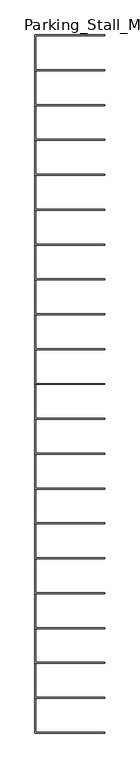
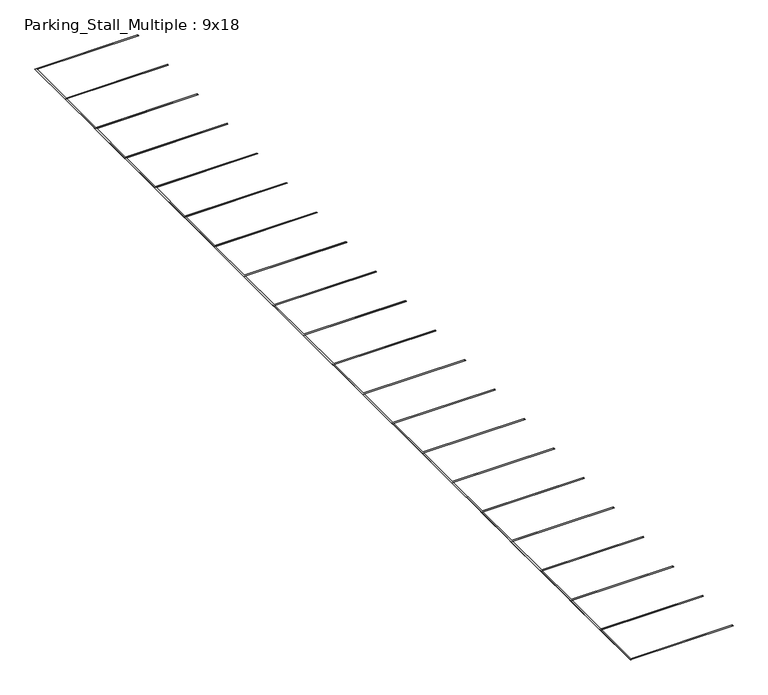
"""IFC4 building model written with IfcOpenShell, lengths in millimetres: proxy geometry, Parking_Stall_Multiple : 9x18."""

import ifcopenshell
import ifcopenshell.guid

model = None  # the IFC model being written
_history = None  # IfcOwnerHistory: only IFC2X3 demands one
_inside = {}  # id of a spatial element -> (the spatial element, [elements in it])
_under = {}  # id of a project, library or spatial element -> (it, [spatial elements below it])
_declared = {}  # id of a project -> (the project, [libraries it declares])
_typed = {}  # id of a type object -> (the type object, [elements of that type])
_made_of = {}  # id of a material, layer set ... -> (it, [elements and type objects made of it])


def new_model(schema):
    """Start an empty IFC model of exactly this schema.

    Asked for "IFC4X3", IfcOpenShell would pick the latest addendum, in which some entities
    have other attributes; the version numbers below select the first issue.
    IFC2X3 requires an IfcOwnerHistory on every rooted entity: one is made here for all.
    """
    global model, _history
    if schema == "IFC4X3":
        model = ifcopenshell.file(schema_version=(4, 3, 0, 0))
    else:
        model = ifcopenshell.file(schema=schema)
    _inside.clear()
    _under.clear()
    _declared.clear()
    _typed.clear()
    _made_of.clear()
    _history = None
    if model.schema == "IFC2X3":
        org = make("IfcOrganization", Name="unknown")
        user = make(
            "IfcPersonAndOrganization",
            ThePerson=make("IfcPerson", FamilyName="unknown"),
            TheOrganization=org,
        )
        app = make(
            "IfcApplication",
            ApplicationDeveloper=org,
            Version="unknown",
            ApplicationFullName="unknown",
            ApplicationIdentifier="unknown",
        )
        _history = make(
            "IfcOwnerHistory",
            OwningUser=user,
            OwningApplication=app,
            ChangeAction="ADDED",
            CreationDate=0,
        )
    return model


def make(cls, **values):
    """One entity of the class cls with the attributes given. An attribute that is None is left unset."""
    return model.create_entity(
        cls, **{name: value for name, value in values.items() if value is not None}
    )


def rooted(cls, **values):
    """An entity with a GlobalId (a new one), such as an element, a storey or a relation."""
    return make(cls, GlobalId=ifcopenshell.guid.new(), OwnerHistory=_history, **values)


def si_unit(unit_type, name, prefix=None):
    """IfcSIUnit, for example si_unit("LENGTHUNIT", "METRE", prefix="MILLI")."""
    return make("IfcSIUnit", UnitType=unit_type, Prefix=prefix, Name=name)


def assignment(units):
    """IfcUnitAssignment: the units of a project."""
    return None if units is None else make("IfcUnitAssignment", Units=units)


def point(xyz):
    """IfcCartesianPoint."""
    return None if xyz is None else make("IfcCartesianPoint", Coordinates=xyz)


def direction(xyz):
    """IfcDirection."""
    return None if xyz is None else make("IfcDirection", DirectionRatios=xyz)


def frame(location, z_axis=None, x_axis=None):
    """IfcAxis2Placement3D, a coordinate frame: its origin and axes. An axis left out is left unset."""
    return make(
        "IfcAxis2Placement3D",
        Location=point(location),
        Axis=direction(z_axis),
        RefDirection=direction(x_axis),
    )


def origin():
    """The frame at (0, 0, 0) with its axes left unset."""
    return frame((0.0, 0.0, 0.0))


def origin_with_axes():
    """The frame at (0, 0, 0) with the z axis (0, 0, 1) and the x axis (1, 0, 0) written out."""
    return frame((0.0, 0.0, 0.0), z_axis=(0.0, 0.0, 1.0), x_axis=(1.0, 0.0, 0.0))


def place(relative_to, where):
    """IfcLocalPlacement: puts the frame where relative to a parent placement (None: the world)."""
    return make(
        "IfcLocalPlacement", PlacementRelTo=relative_to, RelativePlacement=where
    )


def context(
    kind, dimensions, precision=None, world=None, true_north=None, identifier=None
):
    """IfcGeometricRepresentationContext, for example the 3D "Model" context."""
    return make(
        "IfcGeometricRepresentationContext",
        ContextIdentifier=identifier,
        ContextType=kind,
        CoordinateSpaceDimension=dimensions,
        Precision=precision,
        WorldCoordinateSystem=world,
        TrueNorth=true_north,
    )


def project(units=None, contexts=None):
    """IfcProject with its units and contexts."""
    return rooted(
        "IfcProject",
        Name="project",
        RepresentationContexts=contexts,
        UnitsInContext=assignment(units),
    )


def spatial(cls, under=None, at=None, **own):
    """A site, building, storey or space (cls), placed at a placement, below another one or the project."""
    s = rooted(cls, ObjectPlacement=at, **own)
    if under is not None:
        _under.setdefault(under.id(), (under, []))[1].append(s)
    return s


def polyline(points):
    """IfcPolyline through the points."""
    return make("IfcPolyline", Points=[point(p) for p in points])


def outline(outer, holes=None, kind="AREA"):
    """IfcArbitraryClosedProfileDef: a profile drawn as a closed curve; with holes, ...WithVoids."""
    if holes is None:
        return make("IfcArbitraryClosedProfileDef", ProfileType=kind, OuterCurve=outer)
    return make(
        "IfcArbitraryProfileDefWithVoids",
        ProfileType=kind,
        OuterCurve=outer,
        InnerCurves=holes,
    )


def extrude(swept, where, along, depth):
    """IfcExtrudedAreaSolid: the profile swept, set in the frame where, extruded along a direction by depth."""
    return make(
        "IfcExtrudedAreaSolid",
        SweptArea=swept,
        Position=where,
        ExtrudedDirection=direction(along),
        Depth=depth,
    )


def shape(context_of_items, identifier, shape_type, items):
    """IfcShapeRepresentation: the items that make up one representation, for example the "Body"."""
    return make(
        "IfcShapeRepresentation",
        ContextOfItems=context_of_items,
        RepresentationIdentifier=identifier,
        RepresentationType=shape_type,
        Items=items,
    )


def source(mapping_origin, context_of_items, identifier, shape_type, items):
    """IfcRepresentationMap: a shape defined once, which mapped items show again and again."""
    return make(
        "IfcRepresentationMap",
        MappingOrigin=mapping_origin,
        MappedRepresentation=shape(context_of_items, identifier, shape_type, items),
    )


def transform(
    local_origin,
    x_axis=None,
    y_axis=None,
    z_axis=None,
    scale=None,
    scale2=None,
    scale3=None,
    uniform=True,
):
    """IfcCartesianTransformationOperator3D, or its non-uniform kind. x_axis, y_axis, z_axis: its Axis1, 2, 3."""
    if uniform:
        return make(
            "IfcCartesianTransformationOperator3D",
            Axis1=direction(x_axis),
            Axis2=direction(y_axis),
            LocalOrigin=point(local_origin),
            Scale=scale,
            Axis3=direction(z_axis),
        )
    return make(
        "IfcCartesianTransformationOperator3DnonUniform",
        Axis1=direction(x_axis),
        Axis2=direction(y_axis),
        LocalOrigin=point(local_origin),
        Scale=scale,
        Axis3=direction(z_axis),
        Scale2=scale2,
        Scale3=scale3,
    )


def mapped(mapping_source, mapping_target):
    """IfcMappedItem: shows the shape of a source again, moved by a transform."""
    return make(
        "IfcMappedItem", MappingSource=mapping_source, MappingTarget=mapping_target
    )


def made_of(thing, what):
    """Note that an element or type object is made of a material, layer set ...; save() writes the relation."""
    if what is not None:
        _made_of.setdefault(what.id(), (what, []))[1].append(thing)
    return thing


def element(
    cls,
    number,
    at=None,
    inside=None,
    cuts=None,
    type_object=None,
    material=None,
    context=None,
    identifier="Body",
    shape_type=None,
    held_by="IfcProductDefinitionShape",
    body=None,
    shapes=None,
    **own,
):
    """One element of the class cls, such as IfcWall. Its Tag is "e" and its number.

    at: its placement. inside: the storey or other place that contains it. cuts: it is an
    opening in that element (IfcRelVoidsElement). A single representation is given by context,
    identifier, shape_type and body (its items); several are given by shapes. held_by: the class
    of the entity that holds the representations. save() writes the other relations.
    """
    e = rooted(cls, Tag="e%d" % number, ObjectPlacement=at, **own)
    if body is not None:
        shapes = [shape(context, identifier, shape_type, body)]
    if shapes is not None:
        e.Representation = make(held_by, Representations=shapes)
    if inside is not None:
        _inside.setdefault(inside.id(), (inside, []))[1].append(e)
    if cuts is not None:
        rooted(
            "IfcRelVoidsElement", RelatingBuildingElement=cuts, RelatedOpeningElement=e
        )
    if type_object is not None:
        _typed.setdefault(type_object.id(), (type_object, []))[1].append(e)
    return made_of(e, material)


def aggregate(whole, parts):
    """IfcRelAggregates: a whole, such as a stair, and the parts it consists of."""
    return rooted("IfcRelAggregates", RelatingObject=whole, RelatedObjects=parts)


def save(model, path):
    """Write the relations noted so far, then the file.

    IfcRelAggregates (storeys below a building ...), IfcRelContainedInSpatialStructure (elements
    in a storey), IfcRelDefinesByType, IfcRelAssociatesMaterial and IfcRelDeclares: one each for
    every whole, place, type object, material and project.
    """
    for whole, parts in _under.values():
        aggregate(whole, parts)
    for where, things in _inside.values():
        rooted(
            "IfcRelContainedInSpatialStructure",
            RelatedElements=things,
            RelatingStructure=where,
        )
    for kind, things in _typed.values():
        rooted("IfcRelDefinesByType", RelatedObjects=things, RelatingType=kind)
    for what, things in _made_of.values():
        rooted("IfcRelAssociatesMaterial", RelatedObjects=things, RelatingMaterial=what)
    for by, libraries in _declared.values():
        rooted("IfcRelDeclares", RelatingContext=by, RelatedDefinitions=libraries)
    model.write(path)


def parking_stall_multiple_9x18_07dae38a(model_context):
    return source(origin(), model_context, "Body", "SweptSolid", [
        extrude(outline(polyline([(5486.4, 52120.8), (0.0, 52120.8), (0.0, 54940.2), (5486.4, 54940.2), (5486.4, 54864.0), (76.2, 54864.0), (76.2, 52197.0), (5486.4, 52197.0), (5486.4, 52120.8)])), origin_with_axes(), (0.0, 0.0, 1.0), 6.35),
        extrude(outline(polyline([(5486.4, 49377.6), (0.0, 49377.6), (0.0, 52197.0), (5486.4, 52197.0), (5486.4, 52120.8), (76.2, 52120.8), (76.2, 49453.8), (5486.4, 49453.8), (5486.4, 49377.6)])), origin_with_axes(), (0.0, 0.0, 1.0), 6.35),
        extrude(outline(polyline([(5486.4, 46634.4), (0.0, 46634.4), (0.0, 49453.8), (5486.4, 49453.8), (5486.4, 49377.6), (76.2, 49377.6), (76.2, 46710.6), (5486.4, 46710.6), (5486.4, 46634.4)])), origin_with_axes(), (0.0, 0.0, 1.0), 6.35),
        extrude(outline(polyline([(5486.4, 43891.2), (0.0, 43891.2), (0.0, 46710.6), (5486.4, 46710.6), (5486.4, 46634.4), (76.2, 46634.4), (76.2, 43967.4), (5486.4, 43967.4), (5486.4, 43891.2)])), origin_with_axes(), (0.0, 0.0, 1.0), 6.35),
        extrude(outline(polyline([(5486.4, 41148.0), (0.0, 41148.0), (0.0, 43967.4), (5486.4, 43967.4), (5486.4, 43891.2), (76.2, 43891.2), (76.2, 41224.2), (5486.4, 41224.2), (5486.4, 41148.0)])), origin_with_axes(), (0.0, 0.0, 1.0), 6.35),
        extrude(outline(polyline([(5486.4, 38404.8), (0.0, 38404.8), (0.0, 41224.2), (5486.4, 41224.2), (5486.4, 41148.0), (76.2, 41148.0), (76.2, 38481.0), (5486.4, 38481.0), (5486.4, 38404.8)])), origin_with_axes(), (0.0, 0.0, 1.0), 6.35),
        extrude(outline(polyline([(5486.4, 35661.6), (0.0, 35661.6), (0.0, 38481.0), (5486.4, 38481.0), (5486.4, 38404.8), (76.2, 38404.8), (76.2, 35737.8), (5486.4, 35737.8), (5486.4, 35661.6)])), origin_with_axes(), (0.0, 0.0, 1.0), 6.35),
        extrude(outline(polyline([(5486.4, 32918.4), (0.0, 32918.4), (0.0, 35737.8), (5486.4, 35737.8), (5486.4, 35661.6), (76.2, 35661.6), (76.2, 32994.6), (5486.4, 32994.6), (5486.4, 32918.4)])), origin_with_axes(), (0.0, 0.0, 1.0), 6.35),
        extrude(outline(polyline([(5486.4, 30175.2), (0.0, 30175.2), (0.0, 32994.6), (5486.4, 32994.6), (5486.4, 32918.4), (76.2, 32918.4), (76.2, 30251.4), (5486.4, 30251.4), (5486.4, 30175.2)])), origin_with_axes(), (0.0, 0.0, 1.0), 6.35),
        extrude(outline(polyline([(5486.4, 27432.0), (0.0, 27432.0), (0.0, 30251.4), (5486.4, 30251.4), (5486.4, 30175.2), (76.2, 30175.2), (76.2, 27508.2), (5486.4, 27508.2), (5486.4, 27432.0)])), origin_with_axes(), (0.0, 0.0, 1.0), 6.35),
        extrude(outline(polyline([(5486.4, 24688.8), (0.0, 24688.8), (0.0, 27508.2), (5486.4, 27508.2), (5486.4, 27432.0), (76.2, 27432.0), (76.2, 24765.0), (5486.4, 24765.0), (5486.4, 24688.8)])), origin_with_axes(), (0.0, 0.0, 1.0), 6.35),
        extrude(outline(polyline([(5486.4, 21945.6), (0.0, 21945.6), (0.0, 24765.0), (5486.4, 24765.0), (5486.4, 24688.8), (76.2, 24688.8), (76.2, 22021.8), (5486.4, 22021.8), (5486.4, 21945.6)])), origin_with_axes(), (0.0, 0.0, 1.0), 6.35),
        extrude(outline(polyline([(5486.4, 19202.4), (0.0, 19202.4), (0.0, 22021.8), (5486.4, 22021.8), (5486.4, 21945.6), (76.2, 21945.6), (76.2, 19278.6), (5486.4, 19278.6), (5486.4, 19202.4)])), origin_with_axes(), (0.0, 0.0, 1.0), 6.35),
        extrude(outline(polyline([(5486.4, 16459.2), (0.0, 16459.2), (0.0, 19278.6), (5486.4, 19278.6), (5486.4, 19202.4), (76.2, 19202.4), (76.2, 16535.4), (5486.4, 16535.4), (5486.4, 16459.2)])), origin_with_axes(), (0.0, 0.0, 1.0), 6.35),
        extrude(outline(polyline([(5486.4, 13716.0), (0.0, 13716.0), (0.0, 16535.4), (5486.4, 16535.4), (5486.4, 16459.2), (76.2, 16459.2), (76.2, 13792.2), (5486.4, 13792.2), (5486.4, 13716.0)])), origin_with_axes(), (0.0, 0.0, 1.0), 6.35),
        extrude(outline(polyline([(5486.4, 10972.8), (0.0, 10972.8), (0.0, 13792.2), (5486.4, 13792.2), (5486.4, 13716.0), (76.2, 13716.0), (76.2, 11049.0), (5486.4, 11049.0), (5486.4, 10972.8)])), origin_with_axes(), (0.0, 0.0, 1.0), 6.35),
        extrude(outline(polyline([(5486.4, 8229.6), (0.0, 8229.6), (0.0, 11049.0), (5486.4, 11049.0), (5486.4, 10972.8), (76.2, 10972.8), (76.2, 8305.8), (5486.4, 8305.8), (5486.4, 8229.6)])), origin_with_axes(), (0.0, 0.0, 1.0), 6.35),
        extrude(outline(polyline([(5486.4, 5486.4), (0.0, 5486.4), (0.0, 8305.8), (5486.4, 8305.8), (5486.4, 8229.6), (76.2, 8229.6), (76.2, 5562.6), (5486.4, 5562.6), (5486.4, 5486.4)])), origin_with_axes(), (0.0, 0.0, 1.0), 6.35),
        extrude(outline(polyline([(5486.4, 2743.2), (0.0, 2743.2), (0.0, 5562.6), (5486.4, 5562.6), (5486.4, 5486.4), (76.2, 5486.4), (76.2, 2819.4), (5486.4, 2819.4), (5486.4, 2743.2)])), origin_with_axes(), (0.0, 0.0, 1.0), 6.35),
        extrude(outline(polyline([(5486.4, 0.0), (0.0, 0.0), (0.0, 2819.4), (5486.4, 2819.4), (5486.4, 2743.2), (76.2, 2743.2), (76.2, 76.2), (5486.4, 76.2), (5486.4, 0.0)])), origin_with_axes(), (0.0, 0.0, 1.0), 6.35),
    ])


if __name__ == "__main__":
    model = new_model("IFC4")
    model_context = context("Model", 3, world=origin())
    ifc_project = project(units=[si_unit("LENGTHUNIT", "METRE", prefix="MILLI")], contexts=[model_context])
    site = spatial("IfcSite", under=ifc_project)
    building = spatial("IfcBuilding", under=site)
    placement = place(None, origin())
    parking_stall_multiple_9x18_shape = parking_stall_multiple_9x18_07dae38a(model_context)
    element("IfcBuildingElementProxy", 1, Name="Parking_Stall_Multiple : 9x18", ObjectType="Parking_Stall_Multiple : 9x18", at=placement, inside=building, context=model_context, shape_type="MappedRepresentation", body=[
        mapped(parking_stall_multiple_9x18_shape, transform((0.0, 0.0, 0.0), x_axis=(1.0, 0.0, 0.0), y_axis=(0.0, 1.0, 0.0), z_axis=(0.0, 0.0, 1.0))),
    ])
    save(model, "model.ifc")

# Revit data of these elements
# Type "Parking_Stall_Multiple : 9x18"
#   Parking_Width_M = 9' - 0"
#   Parking_Run_Length [instance default] = 65' - 0"
#   Parking_Line_Width = 0' - 3"
#   Parking_Length_M = 18' - 0"
#   Single_Parking_Visibility [instance default] = no
#   Parking_ADA_Symbol = no
#   ParkingUnitsArray [instance default] = 7
#   ParkingUnits [instance default] = 7
#   Multiple_Parking_Visibility [instance default] = yes
#   Parking_Line_Material = none
# Element 1 (IfcBuildingElementProxy, "Parking_Stall_Multiple : 9x18")
#   Parking_Run_Length = 181' - 2.08781"
#   ParkingUnitsArray = 20
#   ParkingUnits = 20
